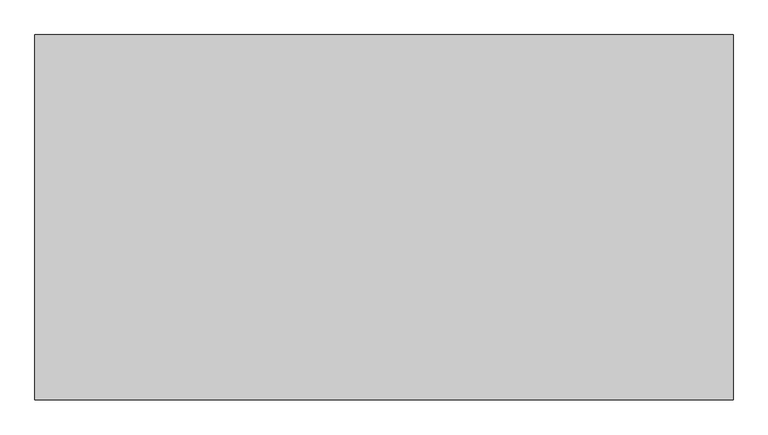
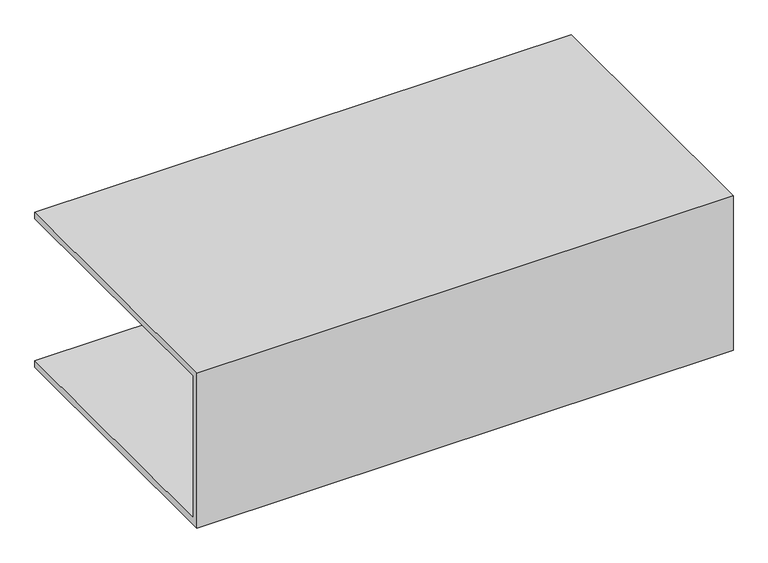
"""IFC4 building model written with IfcOpenShell, lengths in millimetres: proxy geometry, Gypsum024 35614 : Gypsum024 35614."""

from ifc_helpers import new_model, si_unit, frame, origin, place, context, project, spatial, polyline, outline, extrude, source, transform, mapped, element, save


def generic_models_f6582805(model_context):
    return source(origin(), model_context, "Body", "SweptSolid", [
        extrude(outline(polyline([(3440.5759277, 40138.0976562), (3440.5759277, 39579.2929688), (4461.9707031, 39579.2929688), (4461.9707031, 39553.89591), (3415.1759367, 39553.89591), (3415.1759367, 40163.4959196), (4461.9707031, 40163.4959196), (4461.9707031, 40138.0976562), (3440.5759277, 40138.0976562)])), frame((255.0171875, 0.0, 0.0), z_axis=(1.0, 0.0, 0.0), x_axis=(0.0, 1.0, 0.0)), (0.0, 0.0, 1.0), 1999.85),
    ])


if __name__ == "__main__":
    model = new_model("IFC4")
    model_context = context("Model", 3, world=origin())
    ifc_project = project(units=[si_unit("LENGTHUNIT", "METRE", prefix="MILLI")], contexts=[model_context])
    site = spatial("IfcSite", under=ifc_project)
    building = spatial("IfcBuilding", under=site)
    placement = place(None, origin())
    generic_models_shape = generic_models_f6582805(model_context)
    element("IfcBuildingElementProxy", 1, Name="Gypsum024 35614 : Gypsum024 35614", ObjectType="Gypsum024 35614 : Gypsum024 35614", at=placement, inside=building, context=model_context, shape_type="MappedRepresentation", body=[
        mapped(generic_models_shape, transform((0.0, 0.0, 0.0), x_axis=(1.0, 0.0, 0.0), y_axis=(0.0, 1.0, 0.0), z_axis=(0.0, 0.0, 1.0))),
    ])
    save(model, "model.ifc")

# Revit data of these elements
# Type "Gypsum024 35614 : Gypsum024 35614"
#   NameOverride = "Gypsum024"
# Element 1 (IfcBuildingElementProxy, "Gypsum024 35614 : Gypsum024 35614")
#   Materials on its faces: "5/8\" GYPSUM BOARD"
# Materials
#   "5/8\" GYPSUM BOARD": class "Unassigned", colour RGB 214 214 214, transparency 0, Cost = 0
